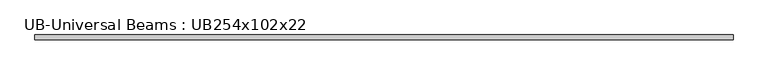
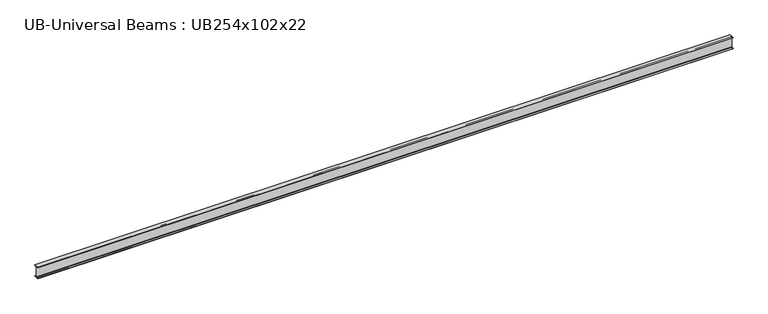
"""IFC4 building model written with IfcOpenShell, lengths in millimetres: beam geometry, UB-Universal Beams : UB254x102x22."""

from ifc_helpers import new_model, si_unit, point, frame, frame_2d, origin, place, context, project, spatial, polyline, circle_curve, trimmed, segment, composite_curve, outline, extrude, source, transform, mapped, element, save


def ub_universal_beams_ub254x102x22_297c9696(model_context):
    return source(origin(), model_context, "Body", "SweptSolid", [
        extrude(outline(composite_curve([segment(polyline([(50.8, -120.2), (50.8, -127.0), (-50.8, -127.0), (-50.8, -120.2), (-10.45, -120.2)]), True, "CONTINUOUS"), segment(trimmed(circle_curve(frame_2d((-10.45, -112.6)), 7.6), [point((-10.45, -120.2))], [point((-2.85, -112.6))], True, "CARTESIAN"), True, "CONTINUOUS"), segment(polyline([(-2.85, -112.6), (-2.85, 112.6)]), True, "CONTINUOUS"), segment(trimmed(circle_curve(frame_2d((-10.45, 112.6)), 7.6), [point((-2.85, 112.6))], [point((-10.45, 120.2))], True, "CARTESIAN"), True, "CONTINUOUS"), segment(polyline([(-10.45, 120.2), (-50.8, 120.2), (-50.8, 127.0), (50.8, 127.0), (50.8, 120.2), (10.45, 120.2)]), True, "CONTINUOUS"), segment(trimmed(circle_curve(frame_2d((10.45, 112.6)), 7.6), [point((10.45, 120.2))], [point((2.85, 112.6))], True, "CARTESIAN"), True, "CONTINUOUS"), segment(polyline([(2.85, 112.6), (2.85, -112.6)]), True, "CONTINUOUS"), segment(trimmed(circle_curve(frame_2d((10.45, -112.6)), 7.6), [point((2.85, -112.6))], [point((10.45, -120.2))], True, "CARTESIAN"), True, "CONTINUOUS"), segment(polyline([(10.45, -120.2), (50.8, -120.2)]), True, "CONTINUOUS")], self_intersect=False)), frame((-7349.2, 0.0, 0.0), z_axis=(1.0, 0.0, 0.0), x_axis=(0.0, 1.0, 0.0)), (0.0, 0.0, 1.0), 14946.35),
    ])


if __name__ == "__main__":
    model = new_model("IFC4")
    model_context = context("Model", 3, world=origin())
    ifc_project = project(units=[si_unit("LENGTHUNIT", "METRE", prefix="MILLI")], contexts=[model_context])
    site = spatial("IfcSite", under=ifc_project)
    building = spatial("IfcBuilding", under=site)
    placement = place(None, origin())
    ub_universal_beams_ub254x102x22_shape = ub_universal_beams_ub254x102x22_297c9696(model_context)
    element("IfcBeam", 1, ObjectType="UB-Universal Beams : UB254x102x22", at=placement, inside=building, context=model_context, shape_type="MappedRepresentation", body=[
        mapped(ub_universal_beams_ub254x102x22_shape, transform((0.0, 0.0, 0.0), x_axis=(1.0, 0.0, 0.0), y_axis=(0.0, 1.0, 0.0), z_axis=(0.0, 0.0, 1.0))),
    ])
    save(model, "model.ifc")

# Revit data of these elements
# Type "UB-Universal Beams : UB254x102x22"
#   Section Name Key = "UB254X102X22"
#   Width = 10.16 cm
#   Web Thickness = 0.57 cm
#   Web Fillet = 0.76 cm
#   Warping Constant = 18200.0 cm⁶
#   Torsional Moment of Inertia = 4.15 cm⁴
#   Section Area = 28.0 cm²
#   Plastic Modulus weak axis = 37.3 cm³
#   Plastic Modulus strong axis = 259.0 cm³
#   Nominal Weight = 22.00 kgf/m
#   Moment of Inertia weak axis = 119.00 cm⁴
#   Moment of Inertia strong axis = 2841.00 cm⁴
#   Height = 25.4 cm
#   Flange Thickness = 0.68 cm
#   Elastic Modulus weak axis = 23.5 cm³
#   Elastic Modulus strong axis = 224.0 cm³
#   Centroid Vertical = 12.7 cm
#   Centroid Horizontal = 5.08 cm
#   Bolt Spacing = 5.4 cm
#   Length [instance default] = 1500 mm
#   Structural Material [instance default] = Metal - Steel 43-275
#   Type Comments = ""
#   Assembly Code = ""
# Element 1 (IfcBeam, "UB-Universal Beams : UB254x102x22")
#   Materials on its faces: "Metal - Steel 43-275"
# Materials
#   "Metal - Steel 43-275": class "Metal", colour RGB 247 247 247, transparency 0, Cost = 0
